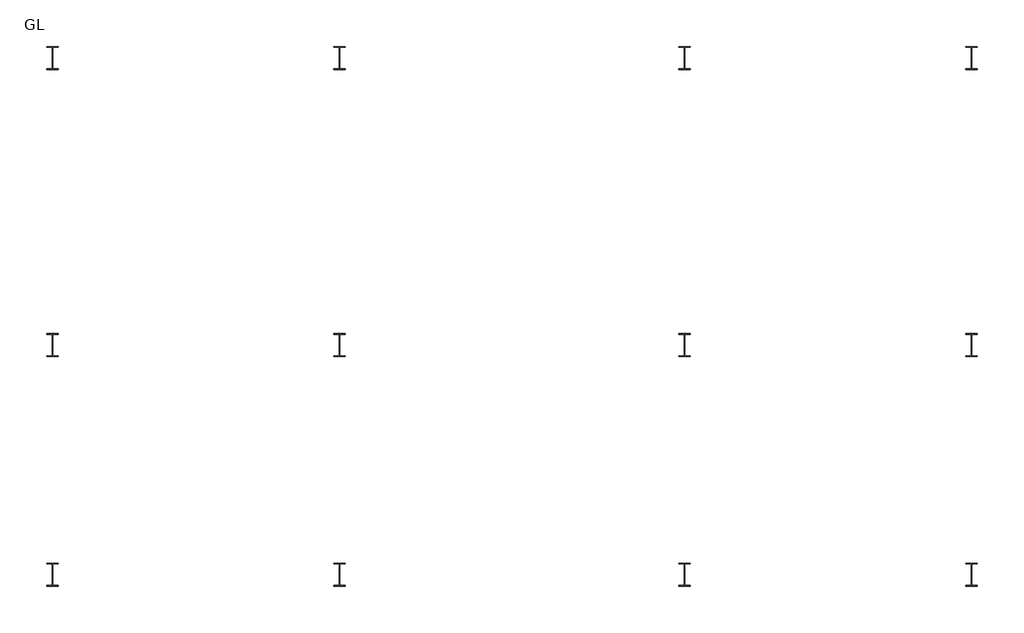
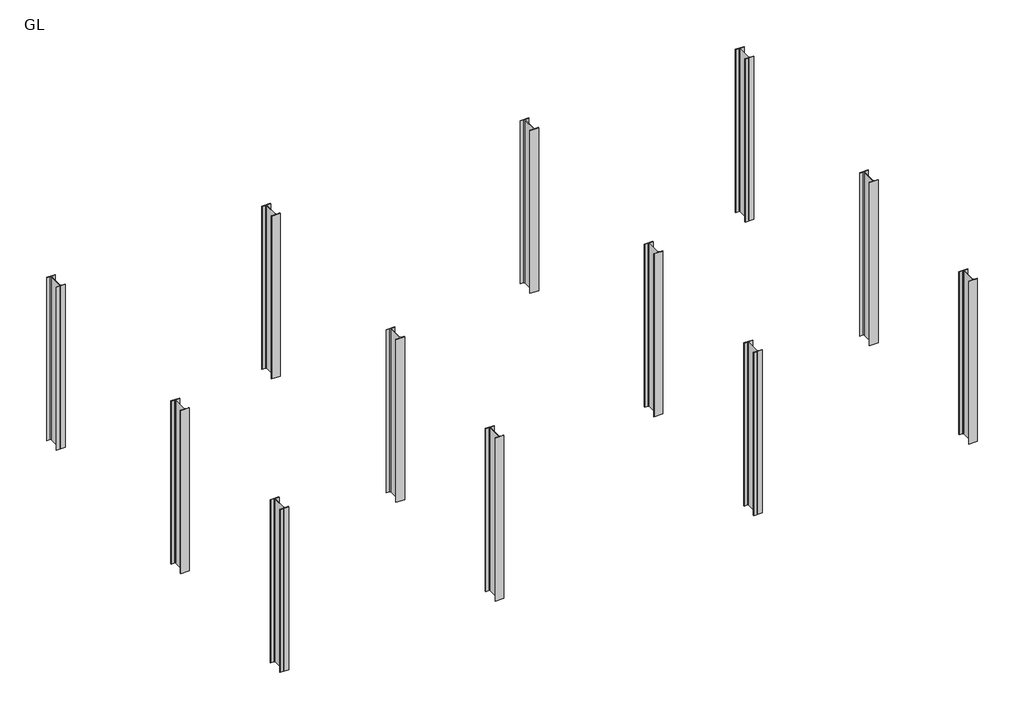
# One storey: 12 columns.
"""IFC4 building model written with IfcOpenShell, lengths in millimetres."""

from ifc_helpers import new_model, si_unit, point, frame_2d, origin, origin_with_axes, place, context, project, spatial, polyline, circle_curve, trimmed, segment, composite_curve, outline, extrude, element, save

model = new_model("IFC4")

# Units and contexts
model_context = context("Model", 3, world=origin())
ifc_project = project(units=[si_unit("LENGTHUNIT", "METRE", prefix="MILLI")], contexts=[model_context])

# Site, building, storey
site = spatial("IfcSite", under=ifc_project)
building = spatial("IfcBuilding", under=site)
storey = spatial("IfcBuildingStorey", under=building, Name="GL", Elevation=-0.0381366)

# Columns
placement = place(None, origin())
element("IfcColumn", 1, ObjectType="Steel Column_H_KSD3502 : H_SC_AR_S01_H-400x200x8x13", at=placement, inside=storey, context=model_context, shape_type="SweptSolid", body=[
    extrude(outline(composite_curve([segment(polyline([(100.0, 200.0), (100.0, 187.0), (20.0, 187.0)]), True, "CONTINUOUS"), segment(trimmed(circle_curve(frame_2d((20.0, 171.0)), 16.0), [point((20.0, 187.0))], [point((4.0, 171.0))], True, "CARTESIAN"), True, "CONTINUOUS"), segment(polyline([(4.0, 171.0), (4.0, -171.0)]), True, "CONTINUOUS"), segment(trimmed(circle_curve(frame_2d((20.0, -171.0)), 16.0), [point((4.0, -171.0))], [point((20.0, -187.0))], True, "CARTESIAN"), True, "CONTINUOUS"), segment(polyline([(20.0, -187.0), (100.0, -187.0), (100.0, -200.0), (-100.0, -200.0), (-100.0, -187.0), (-20.0, -187.0)]), True, "CONTINUOUS"), segment(trimmed(circle_curve(frame_2d((-20.0, -171.0)), 16.0), [point((-20.0, -187.0))], [point((-4.0, -171.0))], True, "CARTESIAN"), True, "CONTINUOUS"), segment(polyline([(-4.0, -171.0), (-4.0, 171.0)]), True, "CONTINUOUS"), segment(trimmed(circle_curve(frame_2d((-20.0, 171.0)), 16.0), [point((-4.0, 171.0))], [point((-20.0, 187.0))], True, "CARTESIAN"), True, "CONTINUOUS"), segment(polyline([(-20.0, 187.0), (-100.0, 187.0), (-100.0, 200.0), (100.0, 200.0)]), True, "CONTINUOUS")], self_intersect=False)), origin_with_axes(), (0.0, 0.0, 1.0), 4000.0),
])
element("IfcColumn", 2, ObjectType="Steel Column_H_KSD3502 : H_SC_AR_S01_H-400x200x8x13", at=placement, inside=storey, context=model_context, shape_type="SweptSolid", body=[
    extrude(outline(composite_curve([segment(polyline([(5100.0, 200.0), (5100.0, 187.0), (5020.0, 187.0)]), True, "CONTINUOUS"), segment(trimmed(circle_curve(frame_2d((5020.0, 171.0)), 16.0), [point((5020.0, 187.0))], [point((5004.0, 171.0))], True, "CARTESIAN"), True, "CONTINUOUS"), segment(polyline([(5004.0, 171.0), (5004.0, -171.0)]), True, "CONTINUOUS"), segment(trimmed(circle_curve(frame_2d((5020.0, -171.0)), 16.0), [point((5004.0, -171.0))], [point((5020.0, -187.0))], True, "CARTESIAN"), True, "CONTINUOUS"), segment(polyline([(5020.0, -187.0), (5100.0, -187.0), (5100.0, -200.0), (4900.0, -200.0), (4900.0, -187.0), (4980.0, -187.0)]), True, "CONTINUOUS"), segment(trimmed(circle_curve(frame_2d((4980.0, -171.0)), 16.0), [point((4980.0, -187.0))], [point((4996.0, -171.0))], True, "CARTESIAN"), True, "CONTINUOUS"), segment(polyline([(4996.0, -171.0), (4996.0, 171.0)]), True, "CONTINUOUS"), segment(trimmed(circle_curve(frame_2d((4980.0, 171.0)), 16.0), [point((4996.0, 171.0))], [point((4980.0, 187.0))], True, "CARTESIAN"), True, "CONTINUOUS"), segment(polyline([(4980.0, 187.0), (4900.0, 187.0), (4900.0, 200.0), (5100.0, 200.0)]), True, "CONTINUOUS")], self_intersect=False)), origin_with_axes(), (0.0, 0.0, 1.0), 4000.0),
])
element("IfcColumn", 3, ObjectType="Steel Column_H_KSD3502 : H_SC_AR_S01_H-400x200x8x13", at=placement, inside=storey, context=model_context, shape_type="SweptSolid", body=[
    extrude(outline(composite_curve([segment(polyline([(11100.0, 200.0), (11100.0, 187.0), (11020.0, 187.0)]), True, "CONTINUOUS"), segment(trimmed(circle_curve(frame_2d((11020.0, 171.0)), 16.0), [point((11020.0, 187.0))], [point((11004.0, 171.0))], True, "CARTESIAN"), True, "CONTINUOUS"), segment(polyline([(11004.0, 171.0), (11004.0, -171.0)]), True, "CONTINUOUS"), segment(trimmed(circle_curve(frame_2d((11020.0, -171.0)), 16.0), [point((11004.0, -171.0))], [point((11020.0, -187.0))], True, "CARTESIAN"), True, "CONTINUOUS"), segment(polyline([(11020.0, -187.0), (11100.0, -187.0), (11100.0, -200.0), (10900.0, -200.0), (10900.0, -187.0), (10980.0, -187.0)]), True, "CONTINUOUS"), segment(trimmed(circle_curve(frame_2d((10980.0, -171.0)), 16.0), [point((10980.0, -187.0))], [point((10996.0, -171.0))], True, "CARTESIAN"), True, "CONTINUOUS"), segment(polyline([(10996.0, -171.0), (10996.0, 171.0)]), True, "CONTINUOUS"), segment(trimmed(circle_curve(frame_2d((10980.0, 171.0)), 16.0), [point((10996.0, 171.0))], [point((10980.0, 187.0))], True, "CARTESIAN"), True, "CONTINUOUS"), segment(polyline([(10980.0, 187.0), (10900.0, 187.0), (10900.0, 200.0), (11100.0, 200.0)]), True, "CONTINUOUS")], self_intersect=False)), origin_with_axes(), (0.0, 0.0, 1.0), 4000.0),
])
element("IfcColumn", 4, ObjectType="Steel Column_H_KSD3502 : H_SC_AR_S01_H-400x200x8x13", at=placement, inside=storey, context=model_context, shape_type="SweptSolid", body=[
    extrude(outline(composite_curve([segment(polyline([(16100.0, 200.0), (16100.0, 187.0), (16020.0, 187.0)]), True, "CONTINUOUS"), segment(trimmed(circle_curve(frame_2d((16020.0, 171.0)), 16.0), [point((16020.0, 187.0))], [point((16004.0, 171.0))], True, "CARTESIAN"), True, "CONTINUOUS"), segment(polyline([(16004.0, 171.0), (16004.0, -171.0)]), True, "CONTINUOUS"), segment(trimmed(circle_curve(frame_2d((16020.0, -171.0)), 16.0), [point((16004.0, -171.0))], [point((16020.0, -187.0))], True, "CARTESIAN"), True, "CONTINUOUS"), segment(polyline([(16020.0, -187.0), (16100.0, -187.0), (16100.0, -200.0), (15900.0, -200.0), (15900.0, -187.0), (15980.0, -187.0)]), True, "CONTINUOUS"), segment(trimmed(circle_curve(frame_2d((15980.0, -171.0)), 16.0), [point((15980.0, -187.0))], [point((15996.0, -171.0))], True, "CARTESIAN"), True, "CONTINUOUS"), segment(polyline([(15996.0, -171.0), (15996.0, 171.0)]), True, "CONTINUOUS"), segment(trimmed(circle_curve(frame_2d((15980.0, 171.0)), 16.0), [point((15996.0, 171.0))], [point((15980.0, 187.0))], True, "CARTESIAN"), True, "CONTINUOUS"), segment(polyline([(15980.0, 187.0), (15900.0, 187.0), (15900.0, 200.0), (16100.0, 200.0)]), True, "CONTINUOUS")], self_intersect=False)), origin_with_axes(), (0.0, 0.0, 1.0), 4000.0),
])
element("IfcColumn", 5, ObjectType="Steel Column_H_KSD3502 : H_SC_AR_S01_H-400x200x8x13", at=placement, inside=storey, context=model_context, shape_type="SweptSolid", body=[
    extrude(outline(composite_curve([segment(polyline([(100.0, 4200.0), (100.0, 4187.0), (20.0, 4187.0)]), True, "CONTINUOUS"), segment(trimmed(circle_curve(frame_2d((20.0, 4171.0)), 16.0), [point((20.0, 4187.0))], [point((4.0, 4171.0))], True, "CARTESIAN"), True, "CONTINUOUS"), segment(polyline([(4.0, 4171.0), (4.0, 3829.0)]), True, "CONTINUOUS"), segment(trimmed(circle_curve(frame_2d((20.0, 3829.0)), 16.0), [point((4.0, 3829.0))], [point((20.0, 3813.0))], True, "CARTESIAN"), True, "CONTINUOUS"), segment(polyline([(20.0, 3813.0), (100.0, 3813.0), (100.0, 3800.0), (-100.0, 3800.0), (-100.0, 3813.0), (-20.0, 3813.0)]), True, "CONTINUOUS"), segment(trimmed(circle_curve(frame_2d((-20.0, 3829.0)), 16.0), [point((-20.0, 3813.0))], [point((-4.0, 3829.0))], True, "CARTESIAN"), True, "CONTINUOUS"), segment(polyline([(-4.0, 3829.0), (-4.0, 4171.0)]), True, "CONTINUOUS"), segment(trimmed(circle_curve(frame_2d((-20.0, 4171.0)), 16.0), [point((-4.0, 4171.0))], [point((-20.0, 4187.0))], True, "CARTESIAN"), True, "CONTINUOUS"), segment(polyline([(-20.0, 4187.0), (-100.0, 4187.0), (-100.0, 4200.0), (100.0, 4200.0)]), True, "CONTINUOUS")], self_intersect=False)), origin_with_axes(), (0.0, 0.0, 1.0), 4000.0),
])
element("IfcColumn", 6, ObjectType="Steel Column_H_KSD3502 : H_SC_AR_S01_H-400x200x8x13", at=placement, inside=storey, context=model_context, shape_type="SweptSolid", body=[
    extrude(outline(composite_curve([segment(polyline([(5100.0, 4200.0), (5100.0, 4187.0), (5020.0, 4187.0)]), True, "CONTINUOUS"), segment(trimmed(circle_curve(frame_2d((5020.0, 4171.0)), 16.0), [point((5020.0, 4187.0))], [point((5004.0, 4171.0))], True, "CARTESIAN"), True, "CONTINUOUS"), segment(polyline([(5004.0, 4171.0), (5004.0, 3829.0)]), True, "CONTINUOUS"), segment(trimmed(circle_curve(frame_2d((5020.0, 3829.0)), 16.0), [point((5004.0, 3829.0))], [point((5020.0, 3813.0))], True, "CARTESIAN"), True, "CONTINUOUS"), segment(polyline([(5020.0, 3813.0), (5100.0, 3813.0), (5100.0, 3800.0), (4900.0, 3800.0), (4900.0, 3813.0), (4980.0, 3813.0)]), True, "CONTINUOUS"), segment(trimmed(circle_curve(frame_2d((4980.0, 3829.0)), 16.0), [point((4980.0, 3813.0))], [point((4996.0, 3829.0))], True, "CARTESIAN"), True, "CONTINUOUS"), segment(polyline([(4996.0, 3829.0), (4996.0, 4171.0)]), True, "CONTINUOUS"), segment(trimmed(circle_curve(frame_2d((4980.0, 4171.0)), 16.0), [point((4996.0, 4171.0))], [point((4980.0, 4187.0))], True, "CARTESIAN"), True, "CONTINUOUS"), segment(polyline([(4980.0, 4187.0), (4900.0, 4187.0), (4900.0, 4200.0), (5100.0, 4200.0)]), True, "CONTINUOUS")], self_intersect=False)), origin_with_axes(), (0.0, 0.0, 1.0), 4000.0),
])
element("IfcColumn", 7, ObjectType="Steel Column_H_KSD3502 : H_SC_AR_S01_H-400x200x8x13", at=placement, inside=storey, context=model_context, shape_type="SweptSolid", body=[
    extrude(outline(composite_curve([segment(polyline([(11100.0, 4200.0), (11100.0, 4187.0), (11020.0, 4187.0)]), True, "CONTINUOUS"), segment(trimmed(circle_curve(frame_2d((11020.0, 4171.0)), 16.0), [point((11020.0, 4187.0))], [point((11004.0, 4171.0))], True, "CARTESIAN"), True, "CONTINUOUS"), segment(polyline([(11004.0, 4171.0), (11004.0, 3829.0)]), True, "CONTINUOUS"), segment(trimmed(circle_curve(frame_2d((11020.0, 3829.0)), 16.0), [point((11004.0, 3829.0))], [point((11020.0, 3813.0))], True, "CARTESIAN"), True, "CONTINUOUS"), segment(polyline([(11020.0, 3813.0), (11100.0, 3813.0), (11100.0, 3800.0), (10900.0, 3800.0), (10900.0, 3813.0), (10980.0, 3813.0)]), True, "CONTINUOUS"), segment(trimmed(circle_curve(frame_2d((10980.0, 3829.0)), 16.0), [point((10980.0, 3813.0))], [point((10996.0, 3829.0))], True, "CARTESIAN"), True, "CONTINUOUS"), segment(polyline([(10996.0, 3829.0), (10996.0, 4171.0)]), True, "CONTINUOUS"), segment(trimmed(circle_curve(frame_2d((10980.0, 4171.0)), 16.0), [point((10996.0, 4171.0))], [point((10980.0, 4187.0))], True, "CARTESIAN"), True, "CONTINUOUS"), segment(polyline([(10980.0, 4187.0), (10900.0, 4187.0), (10900.0, 4200.0), (11100.0, 4200.0)]), True, "CONTINUOUS")], self_intersect=False)), origin_with_axes(), (0.0, 0.0, 1.0), 4000.0),
])
element("IfcColumn", 8, ObjectType="Steel Column_H_KSD3502 : H_SC_AR_S01_H-400x200x8x13", at=placement, inside=storey, context=model_context, shape_type="SweptSolid", body=[
    extrude(outline(composite_curve([segment(polyline([(16100.0, 4200.0), (16100.0, 4187.0), (16020.0, 4187.0)]), True, "CONTINUOUS"), segment(trimmed(circle_curve(frame_2d((16020.0, 4171.0)), 16.0), [point((16020.0, 4187.0))], [point((16004.0, 4171.0))], True, "CARTESIAN"), True, "CONTINUOUS"), segment(polyline([(16004.0, 4171.0), (16004.0, 3829.0)]), True, "CONTINUOUS"), segment(trimmed(circle_curve(frame_2d((16020.0, 3829.0)), 16.0), [point((16004.0, 3829.0))], [point((16020.0, 3813.0))], True, "CARTESIAN"), True, "CONTINUOUS"), segment(polyline([(16020.0, 3813.0), (16100.0, 3813.0), (16100.0, 3800.0), (15900.0, 3800.0), (15900.0, 3813.0), (15980.0, 3813.0)]), True, "CONTINUOUS"), segment(trimmed(circle_curve(frame_2d((15980.0, 3829.0)), 16.0), [point((15980.0, 3813.0))], [point((15996.0, 3829.0))], True, "CARTESIAN"), True, "CONTINUOUS"), segment(polyline([(15996.0, 3829.0), (15996.0, 4171.0)]), True, "CONTINUOUS"), segment(trimmed(circle_curve(frame_2d((15980.0, 4171.0)), 16.0), [point((15996.0, 4171.0))], [point((15980.0, 4187.0))], True, "CARTESIAN"), True, "CONTINUOUS"), segment(polyline([(15980.0, 4187.0), (15900.0, 4187.0), (15900.0, 4200.0), (16100.0, 4200.0)]), True, "CONTINUOUS")], self_intersect=False)), origin_with_axes(), (0.0, 0.0, 1.0), 4000.0),
])
element("IfcColumn", 9, ObjectType="Steel Column_H_KSD3502 : H_SC_AR_S01_H-400x200x8x13", at=placement, inside=storey, context=model_context, shape_type="SweptSolid", body=[
    extrude(outline(composite_curve([segment(polyline([(100.0, 9200.0), (100.0, 9187.0), (20.0, 9187.0)]), True, "CONTINUOUS"), segment(trimmed(circle_curve(frame_2d((20.0, 9171.0)), 16.0), [point((20.0, 9187.0))], [point((4.0, 9171.0))], True, "CARTESIAN"), True, "CONTINUOUS"), segment(polyline([(4.0, 9171.0), (4.0, 8829.0)]), True, "CONTINUOUS"), segment(trimmed(circle_curve(frame_2d((20.0, 8829.0)), 16.0), [point((4.0, 8829.0))], [point((20.0, 8813.0))], True, "CARTESIAN"), True, "CONTINUOUS"), segment(polyline([(20.0, 8813.0), (100.0, 8813.0), (100.0, 8800.0), (-100.0, 8800.0), (-100.0, 8813.0), (-20.0, 8813.0)]), True, "CONTINUOUS"), segment(trimmed(circle_curve(frame_2d((-20.0, 8829.0)), 16.0), [point((-20.0, 8813.0))], [point((-4.0, 8829.0))], True, "CARTESIAN"), True, "CONTINUOUS"), segment(polyline([(-4.0, 8829.0), (-4.0, 9171.0)]), True, "CONTINUOUS"), segment(trimmed(circle_curve(frame_2d((-20.0, 9171.0)), 16.0), [point((-4.0, 9171.0))], [point((-20.0, 9187.0))], True, "CARTESIAN"), True, "CONTINUOUS"), segment(polyline([(-20.0, 9187.0), (-100.0, 9187.0), (-100.0, 9200.0), (100.0, 9200.0)]), True, "CONTINUOUS")], self_intersect=False)), origin_with_axes(), (0.0, 0.0, 1.0), 4000.0),
])
element("IfcColumn", 10, ObjectType="Steel Column_H_KSD3502 : H_SC_AR_S01_H-400x200x8x13", at=placement, inside=storey, context=model_context, shape_type="SweptSolid", body=[
    extrude(outline(composite_curve([segment(polyline([(5100.0, 9200.0), (5100.0, 9187.0), (5020.0, 9187.0)]), True, "CONTINUOUS"), segment(trimmed(circle_curve(frame_2d((5020.0, 9171.0)), 16.0), [point((5020.0, 9187.0))], [point((5004.0, 9171.0))], True, "CARTESIAN"), True, "CONTINUOUS"), segment(polyline([(5004.0, 9171.0), (5004.0, 8829.0)]), True, "CONTINUOUS"), segment(trimmed(circle_curve(frame_2d((5020.0, 8829.0)), 16.0), [point((5004.0, 8829.0))], [point((5020.0, 8813.0))], True, "CARTESIAN"), True, "CONTINUOUS"), segment(polyline([(5020.0, 8813.0), (5100.0, 8813.0), (5100.0, 8800.0), (4900.0, 8800.0), (4900.0, 8813.0), (4980.0, 8813.0)]), True, "CONTINUOUS"), segment(trimmed(circle_curve(frame_2d((4980.0, 8829.0)), 16.0), [point((4980.0, 8813.0))], [point((4996.0, 8829.0))], True, "CARTESIAN"), True, "CONTINUOUS"), segment(polyline([(4996.0, 8829.0), (4996.0, 9171.0)]), True, "CONTINUOUS"), segment(trimmed(circle_curve(frame_2d((4980.0, 9171.0)), 16.0), [point((4996.0, 9171.0))], [point((4980.0, 9187.0))], True, "CARTESIAN"), True, "CONTINUOUS"), segment(polyline([(4980.0, 9187.0), (4900.0, 9187.0), (4900.0, 9200.0), (5100.0, 9200.0)]), True, "CONTINUOUS")], self_intersect=False)), origin_with_axes(), (0.0, 0.0, 1.0), 4000.0),
])
element("IfcColumn", 11, ObjectType="Steel Column_H_KSD3502 : H_SC_AR_S01_H-400x200x8x13", at=placement, inside=storey, context=model_context, shape_type="SweptSolid", body=[
    extrude(outline(composite_curve([segment(polyline([(11100.0, 9200.0), (11100.0, 9187.0), (11020.0, 9187.0)]), True, "CONTINUOUS"), segment(trimmed(circle_curve(frame_2d((11020.0, 9171.0)), 16.0), [point((11020.0, 9187.0))], [point((11004.0, 9171.0))], True, "CARTESIAN"), True, "CONTINUOUS"), segment(polyline([(11004.0, 9171.0), (11004.0, 8829.0)]), True, "CONTINUOUS"), segment(trimmed(circle_curve(frame_2d((11020.0, 8829.0)), 16.0), [point((11004.0, 8829.0))], [point((11020.0, 8813.0))], True, "CARTESIAN"), True, "CONTINUOUS"), segment(polyline([(11020.0, 8813.0), (11100.0, 8813.0), (11100.0, 8800.0), (10900.0, 8800.0), (10900.0, 8813.0), (10980.0, 8813.0)]), True, "CONTINUOUS"), segment(trimmed(circle_curve(frame_2d((10980.0, 8829.0)), 16.0), [point((10980.0, 8813.0))], [point((10996.0, 8829.0))], True, "CARTESIAN"), True, "CONTINUOUS"), segment(polyline([(10996.0, 8829.0), (10996.0, 9171.0)]), True, "CONTINUOUS"), segment(trimmed(circle_curve(frame_2d((10980.0, 9171.0)), 16.0), [point((10996.0, 9171.0))], [point((10980.0, 9187.0))], True, "CARTESIAN"), True, "CONTINUOUS"), segment(polyline([(10980.0, 9187.0), (10900.0, 9187.0), (10900.0, 9200.0), (11100.0, 9200.0)]), True, "CONTINUOUS")], self_intersect=False)), origin_with_axes(), (0.0, 0.0, 1.0), 4000.0),
])
element("IfcColumn", 12, ObjectType="Steel Column_H_KSD3502 : H_SC_AR_S01_H-400x200x8x13", at=placement, inside=storey, context=model_context, shape_type="SweptSolid", body=[
    extrude(outline(composite_curve([segment(polyline([(16100.0, 9200.0), (16100.0, 9187.0), (16020.0, 9187.0)]), True, "CONTINUOUS"), segment(trimmed(circle_curve(frame_2d((16020.0, 9171.0)), 16.0), [point((16020.0, 9187.0))], [point((16004.0, 9171.0))], True, "CARTESIAN"), True, "CONTINUOUS"), segment(polyline([(16004.0, 9171.0), (16004.0, 8829.0)]), True, "CONTINUOUS"), segment(trimmed(circle_curve(frame_2d((16020.0, 8829.0)), 16.0), [point((16004.0, 8829.0))], [point((16020.0, 8813.0))], True, "CARTESIAN"), True, "CONTINUOUS"), segment(polyline([(16020.0, 8813.0), (16100.0, 8813.0), (16100.0, 8800.0), (15900.0, 8800.0), (15900.0, 8813.0), (15980.0, 8813.0)]), True, "CONTINUOUS"), segment(trimmed(circle_curve(frame_2d((15980.0, 8829.0)), 16.0), [point((15980.0, 8813.0))], [point((15996.0, 8829.0))], True, "CARTESIAN"), True, "CONTINUOUS"), segment(polyline([(15996.0, 8829.0), (15996.0, 9171.0)]), True, "CONTINUOUS"), segment(trimmed(circle_curve(frame_2d((15980.0, 9171.0)), 16.0), [point((15996.0, 9171.0))], [point((15980.0, 9187.0))], True, "CARTESIAN"), True, "CONTINUOUS"), segment(polyline([(15980.0, 9187.0), (15900.0, 9187.0), (15900.0, 9200.0), (16100.0, 9200.0)]), True, "CONTINUOUS")], self_intersect=False)), origin_with_axes(), (0.0, 0.0, 1.0), 4000.0),
])

save(model, "model.ifc")

# Revit data of these elements
# Project information
#   H_Seismic Condition = "A as per ASCE 7-10"
#   H_Soil Condition = "C as per ASCE 7-10"
#   H_Basic Wind Speed = "58.3m/s ASCE7-10"
#   H_DS Project Code = "FAASA2302"
#   H_Project Abbreviation = "SACE2"
#   H_Project Division = "화공"
#   H_Project Finish = "2027-03-05"
#   H_Project Location = "Jafurah, Saudi Arabia"
#   H_Project Start = "2024-01-03"
#   H_Project Type = "EPC"
#   H_Smart Code = "FAASA2302"
#   Project Issue Date = "Issue Date"
#   Project Status = "Project Status"
#   Client Name = "Owner"
#   Project Address = "Enter address here"
#   Project Name = "Project Name"
#   Project Number = "0001"
# Grids (mm)
#   "A": line (-3000, 0) -> (19000, 0)
#   "B": line (-3000, 4000) -> (19000, 4000)
#   "C": line (-3000, 9000) -> (19000, 9000)
#   "1": line (0, -3000) -> (0, 12000)
#   "2": line (5000, -3000) -> (5000, 12000)
#   "3": line (11000, -3000) -> (11000, 12000)
#   "4": line (16000, -3000) -> (16000, 12000)
# Type "Steel Column_H_KSD3502 : H_SC_AR_S01_H-400x200x8x13"
#   Width = 20.0 cm
#   Web Thickness = 0.8 cm
#   Web Fillet = 1.6 cm
#   Warping Constant = 648999.0 cm⁶
#   Torsional Moment of Inertia = 35.8981 cm⁴
#   Section Area = 84.12 cm²
#   Plastic Modulus weak axis = 268.0 cm³
#   Plastic Modulus strong axis = 1330.0 cm³
#   Perimeter = 1.56 m²/m
#   Nominal Weight = 66.00 kgf/m
#   Moment of Inertia weak axis = 1740.00 cm⁴
#   Moment of Inertia strong axis = 23700.00 cm⁴
#   Height = 40.0 cm
#   Flange Thickness = 1.3 cm
#   Elastic Modulus weak axis = 174.0 cm³
#   Elastic Modulus strong axis = 1190.0 cm³
#   Centroid Vertical = 20.0 cm
#   Centroid Horizontal = 10.0 cm
#   Structural Material [instance default] = Steel, 45-345
#   Section Name Key = ""
#   Bolt Spacing = 0
#   Assembly Code = ""
# Elements 1, 2, 3, 4, 5, 6, 7, 8, 9, 10, 11, 12 (IfcColumn, "Steel Column_H_KSD3502 : H_SC_AR_S01_H-400x200x8x13")
#   Comments = ""
#   Structural Material = none
#   Phase Created = New Construction
# Materials
#   "Steel, 45-345": class "Metal", colour RGB 189 187 185, transparency 0, Description = "Steel 345 MPa", Cost = 0
